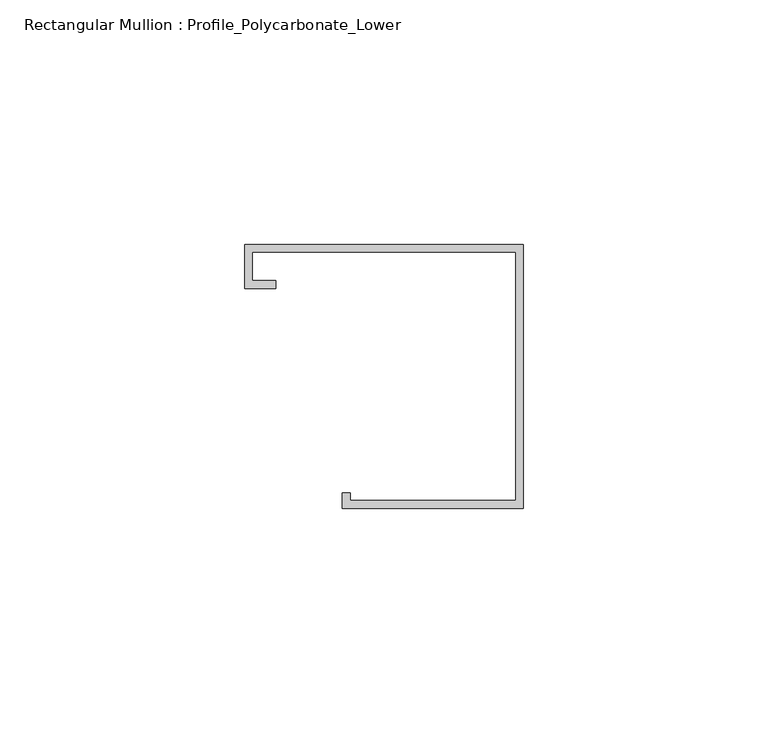
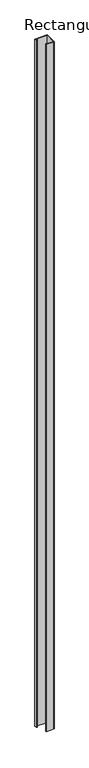
"""IFC4 building model written with IfcOpenShell, lengths in millimetres: member geometry, Rectangular Mullion : Profile_Polycarbonate_Lower."""

from ifc_helpers import new_model, si_unit, frame, origin, place, context, project, spatial, polyline, outline, extrude, source, transform, mapped, element, save


def rectangular_mullion_profile_polycarbonate_lower_41560470(model_context):
    return source(origin(), model_context, "Body", "SweptSolid", [
        extrude(outline(polyline([(0.0, 28.984575), (0.0, -25.015825), (-36.9824, -25.015825), (-36.9824, -21.840825), (-35.3949, -21.840825), (-35.3949, -23.428325), (-1.5875, -23.428325), (-1.5875, 27.397075), (-55.4101, 27.397075), (-55.4101, 21.580475), (-50.6476, 21.580475), (-50.6476, 19.992975), (-56.9976, 19.992975), (-56.9976, 28.984575), (0.0, 28.984575)])), frame((0.0, 0.0, -3346.6024), z_axis=(0.0, 0.0, 1.0), x_axis=(1.0, 0.0, 0.0)), (0.0, 0.0, 1.0), 3346.6024),
    ])


if __name__ == "__main__":
    model = new_model("IFC4")
    model_context = context("Model", 3, world=origin())
    ifc_project = project(units=[si_unit("LENGTHUNIT", "METRE", prefix="MILLI")], contexts=[model_context])
    site = spatial("IfcSite", under=ifc_project)
    building = spatial("IfcBuilding", under=site)
    placement = place(None, origin())
    rectangular_mullion_profile_polycarbonate_lower_shape = rectangular_mullion_profile_polycarbonate_lower_41560470(model_context)
    element("IfcMember", 1, ObjectType="Rectangular Mullion : Profile_Polycarbonate_Lower", at=placement, inside=building, context=model_context, shape_type="MappedRepresentation", body=[
        mapped(rectangular_mullion_profile_polycarbonate_lower_shape, transform((0.0, 0.0, 0.0), x_axis=(1.0, 0.0, 0.0), y_axis=(0.0, 1.0, 0.0), z_axis=(0.0, 0.0, 1.0))),
    ])
    save(model, "model.ifc")

# Revit data of these elements
# Type "Rectangular Mullion : Profile_Polycarbonate_Lower"
#   built-in parameter 1007322 = 0.177167 (stored number, unit not read)
#   built-in parameter 1007321 = 0 (stored number, unit not read)
#   built-in parameter 1007320 = 0.00520833 (stored number, unit not read)
